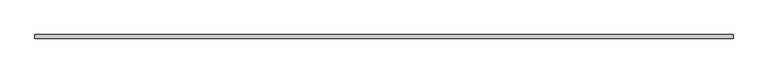
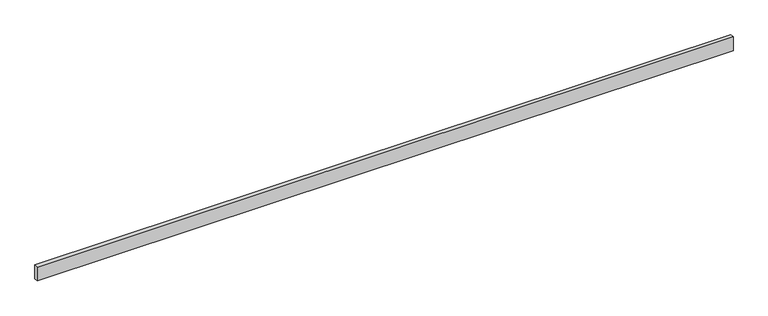
"""IFC4 building model written with IfcOpenShell, lengths in millimetres: proxy geometry, Generic Models 7:Generic Models 1:337419:Generic Models 1:337419 : Generic Models 7:Generic Models 1:337419:19 : Generic Models 7:Generic Models 1:337419:Generic Models 1:337419 : Generic Models 7:Generic Models 1:337419:301336."""

from ifc_helpers import new_model, si_unit, frame, origin, place, context, project, spatial, polyline, outline, extrude, source, transform, mapped, element, save


def generic_models_e323b401(model_context):
    return source(origin(), model_context, "Body", "SweptSolid", [
        extrude(outline(polyline([(596182.8367242, -536531.8913358), (596182.8367242, -536557.2913358), (591306.0367242, -536557.2913358), (591306.0367242, -536531.8913358), (596182.8367242, -536531.8913358)])), frame((0.0, 0.0, 6056.1140625), z_axis=(0.0, 0.0, 1.0), x_axis=(1.0, 0.0, 0.0)), (0.0, 0.0, 1.0), 101.6),
    ])


if __name__ == "__main__":
    model = new_model("IFC4")
    model_context = context("Model", 3, world=origin())
    ifc_project = project(units=[si_unit("LENGTHUNIT", "METRE", prefix="MILLI")], contexts=[model_context])
    site = spatial("IfcSite", under=ifc_project)
    building = spatial("IfcBuilding", under=site)
    placement = place(None, origin())
    generic_models_shape = generic_models_e323b401(model_context)
    element("IfcBuildingElementProxy", 1, Name="Generic Models 7:Generic Models 1:337419:Generic Models 1:337419 : Generic Models 7:Generic Models 1:337419:19 : Generic Models 7:Generic Models 1:337419:Generic Models 1:337419 : Generic Models 7:Generic Models 1:337419:301336", ObjectType="Generic Models 7:Generic Models 1:337419:Generic Models 1:337419 : Generic Models 7:Generic Models 1:337419:19 : Generic Models 7:Generic Models 1:337419:Generic Models 1:337419 : Generic Models 7:Generic Models 1:337419:301336", at=placement, inside=building, context=model_context, shape_type="MappedRepresentation", body=[
        mapped(generic_models_shape, transform((0.0, 0.0, 0.0), x_axis=(1.0, 0.0, 0.0), y_axis=(0.0, 1.0, 0.0), z_axis=(0.0, 0.0, 1.0))),
    ])
    save(model, "model.ifc")

# Revit data of these elements
# Type "Generic Models 7:Generic Models 1:337419:Generic Models 1:337419 : Generic Models 7:Generic Models 1:337419:19 : Generic Models 7:Generic Models 1:337419:Generic Models 1:337419 : Generic Models 7:Generic Models 1:337419:301336"
#   NameOverride = "Generic Models 7:Generic Models 1:337419:Generic Models 1:337419 : Generic Models 7:Generic Models 1:337419:301336"
#   ObjectTypeOverride = "Generic Models 1:337419 : Generic Models 7:Generic Models 1:337419"
#   Reference = "Generic Models 1"
#   Tag = "301336"
# Element 1 (IfcBuildingElementProxy, "Generic Models 7:Generic Models 1:337419:Generic Models 1:337419 : Generic Models 7:Generic Models 1:337419:19 : Generic Models 7:Generic Models 1:337419:Generic Models 1:337419 : Generic Models 7:Generic Models 1:337419:301336")
#   Materials on its faces: "RIGID INSULATION AT GIRTS/JAMB - (CLASS A FLAME SPREAD)"
# Materials
#   "RIGID INSULATION AT GIRTS/JAMB - (CLASS A FLAME SPREAD)": class "Unassigned", colour RGB 205 188 106, transparency 0, Cost = 0
